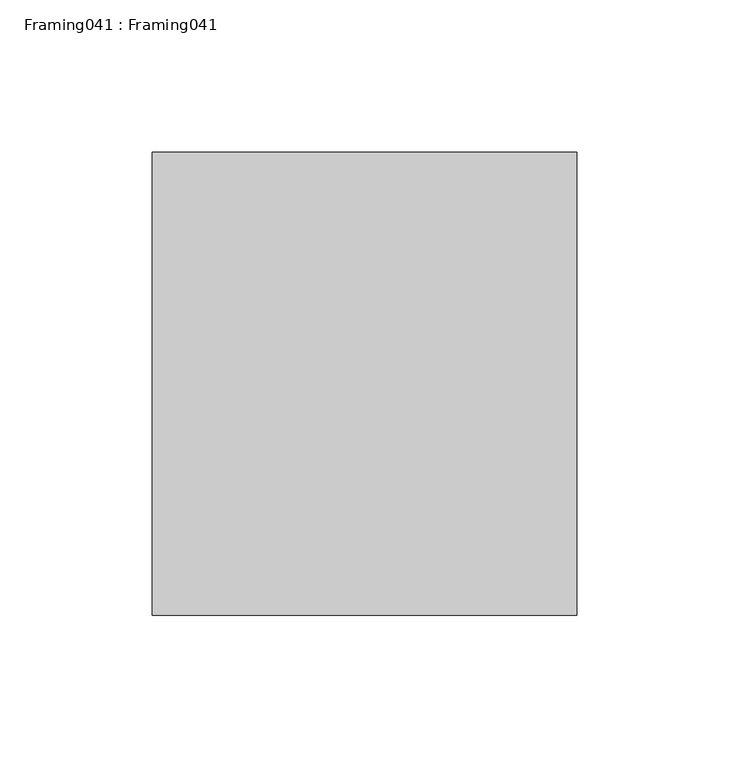
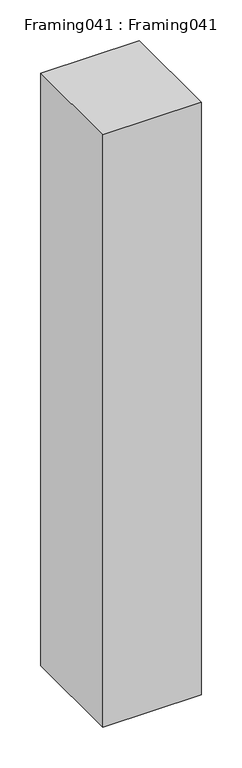
"""IFC4 building model written with IfcOpenShell, lengths in millimetres: proxy geometry, Framing041 : Framing041."""

from ifc_helpers import new_model, si_unit, frame, origin, place, context, project, spatial, polyline, outline, extrude, source, transform, mapped, element, save


def framing041_framing041_e3c462d5(model_context):
    return source(origin(), model_context, "Body", "SweptSolid", [
        extrude(outline(polyline([(-9501.574441, 9829.7529329), (-9641.274441, 9829.7529329), (-9641.274441, 9982.1529329), (-9501.574441, 9982.1529329), (-9501.574441, 9829.7529329)])), frame((0.0, 0.0, 32645.0960433), z_axis=(0.0, 0.0, 1.0), x_axis=(1.0, 0.0, 0.0)), (0.0, 0.0, 1.0), 888.999982),
    ])


if __name__ == "__main__":
    model = new_model("IFC4")
    model_context = context("Model", 3, world=origin())
    ifc_project = project(units=[si_unit("LENGTHUNIT", "METRE", prefix="MILLI")], contexts=[model_context])
    site = spatial("IfcSite", under=ifc_project)
    building = spatial("IfcBuilding", under=site)
    placement = place(None, origin())
    framing041_framing041_shape = framing041_framing041_e3c462d5(model_context)
    element("IfcBuildingElementProxy", 1, Name="Framing041 : Framing041", ObjectType="Framing041 : Framing041", at=placement, inside=building, context=model_context, shape_type="MappedRepresentation", body=[
        mapped(framing041_framing041_shape, transform((0.0, 0.0, 0.0), x_axis=(1.0, 0.0, 0.0), y_axis=(0.0, 1.0, 0.0), z_axis=(0.0, 0.0, 1.0))),
    ])
    save(model, "model.ifc")

# Revit data of these elements
# Type "Framing041 : Framing041"
#   NameOverride = "Framing041"
# Element 1 (IfcBuildingElementProxy, "Framing041 : Framing041")
#   Materials on its faces: "WOOD FRAMING (SEE STRUCT DWGS)"
# Materials
#   "WOOD FRAMING (SEE STRUCT DWGS)": class "Unassigned", colour RGB 224 188 168, transparency 0, Cost = 0
